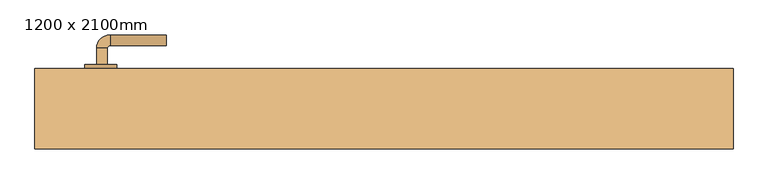
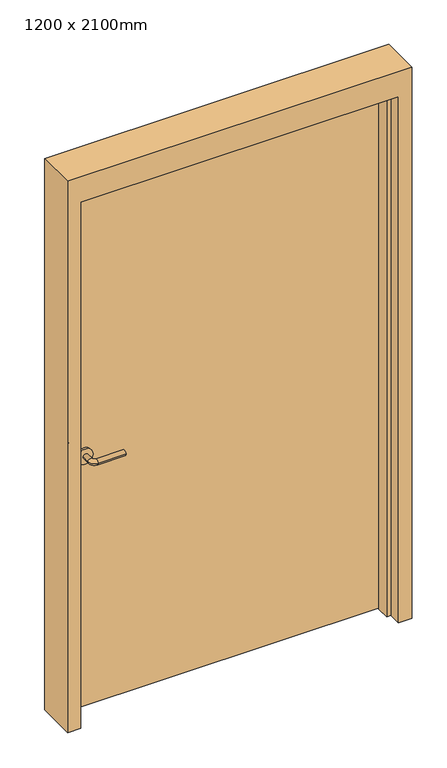
"""IFC4 building model written with IfcOpenShell, lengths in millimetres: door geometry, M_Puerta-De_paso-Simple-Paneles_planos : 1200 x 2100mm."""

from ifc_helpers import new_model, si_unit, point, frame, frame_2d, origin, origin_with_axes, place, context, project, spatial, polyline, circle_curve, ellipse_curve, trimmed, segment, composite_curve, outline, extrude, faceted_brep, source, transform, mapped, element, save
from ifc_brep_helpers import plane_surface, cylinder_surface, revolved_surface, advanced_brep


def door_1200_x_2100mm_adb88274(model_context):
    return source(origin(), model_context, "Body", "SolidModel", [
        advanced_brep(
        [(-534.990625, 3.35, 1000.0), (-514.990625, 3.35, 1000.0), (-514.990625, -26.65, 1000.0), (-534.990625, -26.65, 1000.0), (-509.990625, -31.65, 1000.0), (-509.990625, -51.65, 1000.0), (-404.990625, -51.65, 1000.0), (-404.990625, -31.65, 1000.0)],
        [
            (0, 1, circle_curve(frame((-524.990625, 3.35, 1000.0), z_axis=(0.0, 1.0, 0.0), x_axis=(1.0, 0.0, 0.0)), 10.0)),
            (1, 0, circle_curve(frame((-524.990625, 3.35, 1000.0), z_axis=(0.0, 1.0, 0.0), x_axis=(1.0, 0.0, 0.0)), 10.0)),
            (1, 2),
            (2, 3, circle_curve(frame((-524.990625, -26.65, 1000.0), z_axis=(0.0, 1.0, 0.0), x_axis=(1.0, 0.0, 0.0)), 10.0)),
            (3, 0),
            (3, 2, circle_curve(frame((-524.990625, -26.65, 1000.0), z_axis=(0.0, 1.0, 0.0), x_axis=(1.0, 0.0, 0.0)), 10.0)),
            (4, 5, circle_curve(frame((-509.990625, -41.65, 1000.0), z_axis=(-1.0, 0.0, 0.0), x_axis=(0.0, 1.0, 0.0)), 10.0)),
            (5, 3, circle_curve(frame((-509.990625, -26.65, 1000.0), z_axis=(0.0, 0.0, -1.0), x_axis=(-1.0, 0.0, 0.0)), 25.0)),
            (2, 4, circle_curve(frame((-509.990625, -26.65, 1000.0), z_axis=(0.0, 0.0, 1.0), x_axis=(-1.0, 0.0, 0.0)), 5.0)),
            (5, 4, circle_curve(frame((-509.990625, -41.65, 1000.0), z_axis=(-1.0, 0.0, 0.0), x_axis=(0.0, 1.0, 0.0)), 10.0)),
            (6, 7, circle_curve(frame((-404.990625, -41.65, 1000.0), z_axis=(1.0, 0.0, 0.0), x_axis=(0.0, 1.0, 0.0)), 10.0)),
            (7, 6, circle_curve(frame((-404.990625, -41.65, 1000.0), z_axis=(1.0, 0.0, 0.0), x_axis=(0.0, 1.0, 0.0)), 10.0)),
            (4, 7),
            (6, 5),
        ],
        [
            plane_surface(frame((-524.990625, 3.35, 1000.0), z_axis=(0.0, 1.0, 0.0), x_axis=(0.0, 0.0, 1.0))),
            cylinder_surface(frame((-524.990625, 3.35, 1000.0), z_axis=(0.0, 1.0, 0.0), x_axis=(1.0, 0.0, 0.0)), 10.0),
            revolved_surface(trimmed(ellipse_curve(frame((-524.990625, -26.65, 1000.0), z_axis=(0.0, -1.0, 0.0), x_axis=(1.0, 0.0, 0.0)), 10.0, 10.0), [point((-534.990625, -26.65, 1000.0))], [point((-514.990625, -26.65, 1000.0))], True, "CARTESIAN"), (-509.990625, -26.65, 1000.0), (0.0, 0.0, -1.0)),
            revolved_surface(trimmed(ellipse_curve(frame((-524.990625, -26.65, 1000.0), z_axis=(0.0, -1.0, 0.0), x_axis=(1.0, 0.0, 0.0)), 10.0, 10.0), [point((-514.990625, -26.65, 1000.0))], [point((-534.990625, -26.65, 1000.0))], True, "CARTESIAN"), (-509.990625, -26.65, 1000.0), (0.0, 0.0, -1.0)),
            plane_surface(frame((-404.990625, -41.65, 1000.0), z_axis=(1.0, 0.0, 0.0), x_axis=(0.0, 0.0, 1.0))),
            cylinder_surface(frame((-509.990625, -41.65, 1000.0), z_axis=(-1.0, 0.0, 0.0), x_axis=(0.0, 1.0, 0.0)), 10.0),
        ],
        [
            (0, [[1, 2]]),
            (1, [[3, 4, 5, -2]]),
            (1, [[-5, 6, -3, -1]]),
            (2, [[7, 8, -4, 9]]),
            (3, [[10, -9, -6, -8]]),
            (4, [[11, 12]]),
            (5, [[13, -11, 14, -7]]),
            (5, [[-14, -12, -13, -10]]),
        ],
    ),
        extrude(outline(composite_curve([segment(trimmed(circle_curve(frame_2d((1000.0, -527.490625)), 30.0), [point((1000.0, -557.490625))], [point((1000.0, -497.490625))], False, "CARTESIAN"), True, "CONTINUOUS"), segment(trimmed(circle_curve(frame_2d((1000.0, -527.490625)), 30.0), [point((1000.0, -497.490625))], [point((1000.0, -557.490625))], False, "CARTESIAN"), True, "CONTINUOUS")], self_intersect=False)), frame((0.0, 3.35, 0.0), z_axis=(0.0, 1.0, 0.0), x_axis=(0.0, 0.0, 1.0)), (0.0, 0.0, 1.0), 8.0),
        advanced_brep(
        [(-534.990625, 64.35, 1000.0), (-514.990625, 64.35, 1000.0), (-534.990625, 94.35, 1000.0), (-514.990625, 94.35, 1000.0), (-509.990625, 99.35, 1000.0), (-509.990625, 119.35, 1000.0), (-404.990625, 119.35, 1000.0), (-404.990625, 99.35, 1000.0)],
        [
            (0, 1, circle_curve(frame((-524.990625, 64.35, 1000.0), z_axis=(0.0, -1.0, 0.0), x_axis=(1.0, 0.0, 0.0)), 10.0)),
            (1, 0, circle_curve(frame((-524.990625, 64.35, 1000.0), z_axis=(0.0, -1.0, 0.0), x_axis=(1.0, 0.0, 0.0)), 10.0)),
            (0, 2),
            (2, 3, circle_curve(frame((-524.990625, 94.35, 1000.0), z_axis=(0.0, -1.0, 0.0), x_axis=(1.0, 0.0, 0.0)), 10.0)),
            (3, 1),
            (3, 2, circle_curve(frame((-524.990625, 94.35, 1000.0), z_axis=(0.0, -1.0, 0.0), x_axis=(1.0, 0.0, 0.0)), 10.0)),
            (4, 3, circle_curve(frame((-509.990625, 94.35, 1000.0), z_axis=(0.0, 0.0, 1.0), x_axis=(-1.0, 0.0, 0.0)), 5.0)),
            (2, 5, circle_curve(frame((-509.990625, 94.35, 1000.0), z_axis=(0.0, 0.0, -1.0), x_axis=(-1.0, 0.0, 0.0)), 25.0)),
            (5, 4, circle_curve(frame((-509.990625, 109.35, 1000.0), z_axis=(-1.0, 0.0, 0.0), x_axis=(0.0, -1.0, 0.0)), 10.0)),
            (4, 5, circle_curve(frame((-509.990625, 109.35, 1000.0), z_axis=(-1.0, 0.0, 0.0), x_axis=(0.0, -1.0, 0.0)), 10.0)),
            (6, 7, circle_curve(frame((-404.990625, 109.35, 1000.0), z_axis=(1.0, 0.0, 0.0), x_axis=(0.0, -1.0, 0.0)), 10.0)),
            (7, 6, circle_curve(frame((-404.990625, 109.35, 1000.0), z_axis=(1.0, 0.0, 0.0), x_axis=(0.0, -1.0, 0.0)), 10.0)),
            (5, 6),
            (7, 4),
        ],
        [
            plane_surface(frame((-524.990625, 64.35, 1000.0), z_axis=(0.0, -1.0, 0.0), x_axis=(0.0, 0.0, 1.0))),
            cylinder_surface(frame((-524.990625, 64.35, 1000.0), z_axis=(0.0, -1.0, 0.0), x_axis=(1.0, 0.0, 0.0)), 10.0),
            revolved_surface(trimmed(ellipse_curve(frame((-524.990625, 94.35, 1000.0), z_axis=(0.0, -1.0, 0.0), x_axis=(1.0, 0.0, 0.0)), 10.0, 10.0), [point((-534.990625, 94.35, 1000.0))], [point((-514.990625, 94.35, 1000.0))], True, "CARTESIAN"), (-509.990625, 94.35, 1000.0), (0.0, 0.0, -1.0)),
            revolved_surface(trimmed(ellipse_curve(frame((-524.990625, 94.35, 1000.0), z_axis=(0.0, -1.0, 0.0), x_axis=(1.0, 0.0, 0.0)), 10.0, 10.0), [point((-514.990625, 94.35, 1000.0))], [point((-534.990625, 94.35, 1000.0))], True, "CARTESIAN"), (-509.990625, 94.35, 1000.0), (0.0, 0.0, -1.0)),
            plane_surface(frame((-404.990625, 109.35, 1000.0), z_axis=(1.0, 0.0, 0.0), x_axis=(0.0, 0.0, 1.0))),
            cylinder_surface(frame((-509.990625, 109.35, 1000.0), z_axis=(-1.0, 0.0, 0.0), x_axis=(0.0, -1.0, 0.0)), 10.0),
        ],
        [
            (0, [[1, 2]]),
            (1, [[-1, 3, 4, 5]]),
            (1, [[-2, -5, 6, -3]]),
            (2, [[7, -4, 8, 9]]),
            (3, [[-8, -6, -7, 10]]),
            (4, [[11, 12]]),
            (5, [[-9, 13, -12, 14]]),
            (5, [[-10, -14, -11, -13]]),
        ],
    ),
        extrude(outline(composite_curve([segment(trimmed(circle_curve(frame_2d((1000.0, -527.490625)), 30.0), [point((1000.0, -557.490625))], [point((1000.0, -497.490625))], False, "CARTESIAN"), True, "CONTINUOUS"), segment(trimmed(circle_curve(frame_2d((1000.0, -527.490625)), 30.0), [point((1000.0, -497.490625))], [point((1000.0, -557.490625))], False, "CARTESIAN"), True, "CONTINUOUS")], self_intersect=False)), frame((0.0, 56.35, 0.0), z_axis=(0.0, 1.0, 0.0), x_axis=(0.0, 0.0, 1.0)), (0.0, 0.0, 1.0), 8.0),
        extrude(outline(polyline([(600.0, 11.35), (-600.0, 11.35), (-600.0, 56.35), (600.0, 56.35), (600.0, 11.35)])), origin_with_axes(), (0.0, 0.0, 1.0), 2100.0),
        faceted_brep([(600.0, 6.5875, 0.0), (600.0, 56.35, 0.0), (650.0, 56.35, 0.0), (650.0, -93.65, 0.0), (600.0, -93.65, 0.0), (600.0, -44.4375, 0.0), (584.125, -44.4375, 0.0), (584.125, 6.5875, 0.0), (600.0, 6.5875, 2100.0), (600.0, 56.35, 2100.0), (-600.0, 56.35, 2100.0), (-600.0, 56.35, 0.0), (-650.0, 56.35, 0.0), (-650.0, 56.35, 2200.0), (650.0, 56.35, 2200.0), (650.0, -93.65, 2200.0), (-650.0, -93.65, 2200.0), (-650.0, -93.65, 0.0), (-600.0, -93.65, 0.0), (-600.0, -93.65, 2100.0), (600.0, -93.65, 2100.0), (600.0, -44.4375, 2100.0), (-600.0, -44.4375, 2100.0), (-600.0, -44.4375, 0.0), (-584.125, -44.4375, 0.0), (-584.125, -44.4375, 2084.125), (584.125, -44.4375, 2084.125), (584.125, 6.5875, 2084.125), (-584.125, 6.5875, 2084.125), (-584.125, 6.5875, 0.0), (-600.0, 6.5875, 0.0), (-600.0, 6.5875, 2100.0)], [[[0, 1, 2, 3, 4, 5, 6, 7]], [[1, 0, 8, 9]], [[2, 1, 9, 10, 11, 12, 13, 14]], [[3, 2, 14, 15]], [[4, 3, 15, 16, 17, 18, 19, 20]], [[5, 4, 20, 21]], [[6, 5, 21, 22, 23, 24, 25, 26]], [[7, 6, 26, 27]], [[0, 7, 27, 28, 29, 30, 31, 8]], [[9, 8, 31, 10]], [[20, 19, 22, 21]], [[26, 25, 28, 27]], [[12, 11, 30, 29, 24, 23, 18, 17]], [[11, 10, 31, 30]], [[13, 12, 17, 16]], [[19, 18, 23, 22]], [[25, 24, 29, 28]], [[15, 14, 13, 16]]]),
    ])


if __name__ == "__main__":
    model = new_model("IFC4")
    model_context = context("Model", 3, world=origin())
    ifc_project = project(units=[si_unit("LENGTHUNIT", "METRE", prefix="MILLI")], contexts=[model_context])
    site = spatial("IfcSite", under=ifc_project)
    building = spatial("IfcBuilding", under=site)
    placement = place(None, origin())
    door_1200_x_2100mm_shape = door_1200_x_2100mm_adb88274(model_context)
    element("IfcDoor", 1, ObjectType="M_Puerta-De_paso-Simple-Paneles_planos : 1200 x 2100mm", at=placement, inside=building, context=model_context, shape_type="MappedRepresentation", body=[
        mapped(door_1200_x_2100mm_shape, transform((0.0, 0.0, 0.0), x_axis=(1.0, 0.0, 0.0), y_axis=(0.0, 1.0, 0.0), z_axis=(0.0, 0.0, 1.0))),
    ])
    save(model, "model.ifc")

# Revit data of these elements
# Type "M_Puerta-De_paso-Simple-Paneles_planos : 1200 x 2100mm"
#   Type Mark = "46"
#   Analytic Construction = "Madera"
#   Thickness = 0.045 m
#   Thermal Resistance (R) = 0.455703 (m²·K)/W
#   Ángulo de batiente [instance default] = 90.00°
#   Altura del pasador = 1.00 m
#   Rough Width [instance default] = 1.30 m
#   Rough Height [instance default] = 2.20 m
#   Altura de hueco MF [instance default] = 0.10 m
#   Anchura de hueco MF [instance default] = 0.10 m
#   Cálculo de la incrustación [instance default] = 0.105 m
#   Incrustación de albañilería [instance default] = 0.025 m
#   Height = 2.10 m
#   Width = 1.20 m
#   Heat Transfer Coefficient (U) = 2.19465 W/(m²·K)
#   Profundidad del marco del albañilería = 0.15 m
#   Marco del albañilería [instance default] = yes
#   Function = 1
#   Marco de muro seco [instance default] = no
#   Material de panel = Madera - Abedul
#   Material de estructura = Metal - Acabado de pintura - Gris
#   Material de tirador = Aluminio 1
#   Visual Light Transmittance = 0
#   Solar Heat Gain Coefficient = 0
#   Wall Closure = (empty or 0)
# Element 1 (IfcDoor, "M_Puerta-De_paso-Simple-Paneles_planos : 1200 x 2100mm")
#   Materials on its faces: "Aluminio 1", "Metal - Acabado de pintura - Gris", "Madera - Abedul"
# Materials
#   "Madera - Abedul": class "Madera", colour RGB 173 132 96, transparency 0, Cost = 0
#   "Metal - Acabado de pintura - Gris": class "Pintura", colour RGB 178 178 178, transparency 0, Cost = 0
#   "Aluminio 1": class "Metal", colour RGB 244 245 246, transparency 0, Description = "Aluminio 6061", Cost = 0
